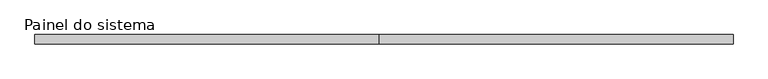
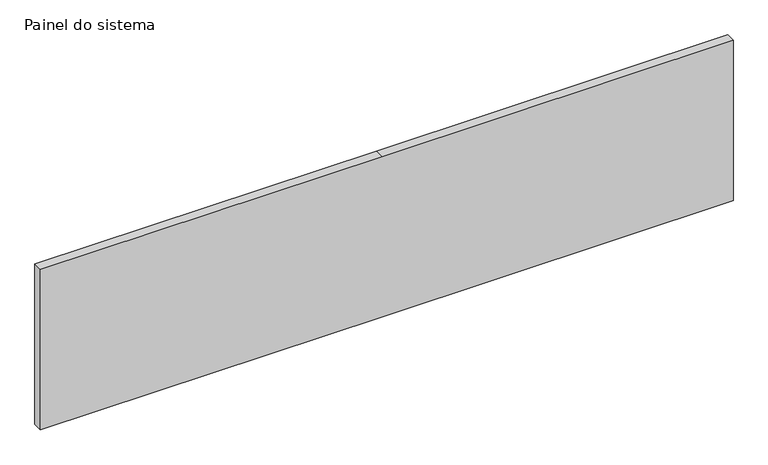
"""IFC4 building model written with IfcOpenShell, lengths in millimetres: plate geometry, Painel do sistema : Envidraçado."""

import ifcopenshell
import ifcopenshell.guid

model = None  # the IFC model being written
_history = None  # IfcOwnerHistory: only IFC2X3 demands one
_inside = {}  # id of a spatial element -> (the spatial element, [elements in it])
_under = {}  # id of a project, library or spatial element -> (it, [spatial elements below it])
_declared = {}  # id of a project -> (the project, [libraries it declares])
_typed = {}  # id of a type object -> (the type object, [elements of that type])
_made_of = {}  # id of a material, layer set ... -> (it, [elements and type objects made of it])


def new_model(schema):
    """Start an empty IFC model of exactly this schema.

    Asked for "IFC4X3", IfcOpenShell would pick the latest addendum, in which some entities
    have other attributes; the version numbers below select the first issue.
    IFC2X3 requires an IfcOwnerHistory on every rooted entity: one is made here for all.
    """
    global model, _history
    if schema == "IFC4X3":
        model = ifcopenshell.file(schema_version=(4, 3, 0, 0))
    else:
        model = ifcopenshell.file(schema=schema)
    _inside.clear()
    _under.clear()
    _declared.clear()
    _typed.clear()
    _made_of.clear()
    _history = None
    if model.schema == "IFC2X3":
        org = make("IfcOrganization", Name="unknown")
        user = make(
            "IfcPersonAndOrganization",
            ThePerson=make("IfcPerson", FamilyName="unknown"),
            TheOrganization=org,
        )
        app = make(
            "IfcApplication",
            ApplicationDeveloper=org,
            Version="unknown",
            ApplicationFullName="unknown",
            ApplicationIdentifier="unknown",
        )
        _history = make(
            "IfcOwnerHistory",
            OwningUser=user,
            OwningApplication=app,
            ChangeAction="ADDED",
            CreationDate=0,
        )
    return model


def make(cls, **values):
    """One entity of the class cls with the attributes given. An attribute that is None is left unset."""
    return model.create_entity(
        cls, **{name: value for name, value in values.items() if value is not None}
    )


def rooted(cls, **values):
    """An entity with a GlobalId (a new one), such as an element, a storey or a relation."""
    return make(cls, GlobalId=ifcopenshell.guid.new(), OwnerHistory=_history, **values)


def si_unit(unit_type, name, prefix=None):
    """IfcSIUnit, for example si_unit("LENGTHUNIT", "METRE", prefix="MILLI")."""
    return make("IfcSIUnit", UnitType=unit_type, Prefix=prefix, Name=name)


def assignment(units):
    """IfcUnitAssignment: the units of a project."""
    return None if units is None else make("IfcUnitAssignment", Units=units)


def point(xyz):
    """IfcCartesianPoint."""
    return None if xyz is None else make("IfcCartesianPoint", Coordinates=xyz)


def direction(xyz):
    """IfcDirection."""
    return None if xyz is None else make("IfcDirection", DirectionRatios=xyz)


def frame(location, z_axis=None, x_axis=None):
    """IfcAxis2Placement3D, a coordinate frame: its origin and axes. An axis left out is left unset."""
    return make(
        "IfcAxis2Placement3D",
        Location=point(location),
        Axis=direction(z_axis),
        RefDirection=direction(x_axis),
    )


def origin():
    """The frame at (0, 0, 0) with its axes left unset."""
    return frame((0.0, 0.0, 0.0))


def place(relative_to, where):
    """IfcLocalPlacement: puts the frame where relative to a parent placement (None: the world)."""
    return make(
        "IfcLocalPlacement", PlacementRelTo=relative_to, RelativePlacement=where
    )


def context(
    kind, dimensions, precision=None, world=None, true_north=None, identifier=None
):
    """IfcGeometricRepresentationContext, for example the 3D "Model" context."""
    return make(
        "IfcGeometricRepresentationContext",
        ContextIdentifier=identifier,
        ContextType=kind,
        CoordinateSpaceDimension=dimensions,
        Precision=precision,
        WorldCoordinateSystem=world,
        TrueNorth=true_north,
    )


def project(units=None, contexts=None):
    """IfcProject with its units and contexts."""
    return rooted(
        "IfcProject",
        Name="project",
        RepresentationContexts=contexts,
        UnitsInContext=assignment(units),
    )


def spatial(cls, under=None, at=None, **own):
    """A site, building, storey or space (cls), placed at a placement, below another one or the project."""
    s = rooted(cls, ObjectPlacement=at, **own)
    if under is not None:
        _under.setdefault(under.id(), (under, []))[1].append(s)
    return s


def polyline(points):
    """IfcPolyline through the points."""
    return make("IfcPolyline", Points=[point(p) for p in points])


def outline(outer, holes=None, kind="AREA"):
    """IfcArbitraryClosedProfileDef: a profile drawn as a closed curve; with holes, ...WithVoids."""
    if holes is None:
        return make("IfcArbitraryClosedProfileDef", ProfileType=kind, OuterCurve=outer)
    return make(
        "IfcArbitraryProfileDefWithVoids",
        ProfileType=kind,
        OuterCurve=outer,
        InnerCurves=holes,
    )


def extrude(swept, where, along, depth):
    """IfcExtrudedAreaSolid: the profile swept, set in the frame where, extruded along a direction by depth."""
    return make(
        "IfcExtrudedAreaSolid",
        SweptArea=swept,
        Position=where,
        ExtrudedDirection=direction(along),
        Depth=depth,
    )


def shape(context_of_items, identifier, shape_type, items):
    """IfcShapeRepresentation: the items that make up one representation, for example the "Body"."""
    return make(
        "IfcShapeRepresentation",
        ContextOfItems=context_of_items,
        RepresentationIdentifier=identifier,
        RepresentationType=shape_type,
        Items=items,
    )


def source(mapping_origin, context_of_items, identifier, shape_type, items):
    """IfcRepresentationMap: a shape defined once, which mapped items show again and again."""
    return make(
        "IfcRepresentationMap",
        MappingOrigin=mapping_origin,
        MappedRepresentation=shape(context_of_items, identifier, shape_type, items),
    )


def transform(
    local_origin,
    x_axis=None,
    y_axis=None,
    z_axis=None,
    scale=None,
    scale2=None,
    scale3=None,
    uniform=True,
):
    """IfcCartesianTransformationOperator3D, or its non-uniform kind. x_axis, y_axis, z_axis: its Axis1, 2, 3."""
    if uniform:
        return make(
            "IfcCartesianTransformationOperator3D",
            Axis1=direction(x_axis),
            Axis2=direction(y_axis),
            LocalOrigin=point(local_origin),
            Scale=scale,
            Axis3=direction(z_axis),
        )
    return make(
        "IfcCartesianTransformationOperator3DnonUniform",
        Axis1=direction(x_axis),
        Axis2=direction(y_axis),
        LocalOrigin=point(local_origin),
        Scale=scale,
        Axis3=direction(z_axis),
        Scale2=scale2,
        Scale3=scale3,
    )


def mapped(mapping_source, mapping_target):
    """IfcMappedItem: shows the shape of a source again, moved by a transform."""
    return make(
        "IfcMappedItem", MappingSource=mapping_source, MappingTarget=mapping_target
    )


def made_of(thing, what):
    """Note that an element or type object is made of a material, layer set ...; save() writes the relation."""
    if what is not None:
        _made_of.setdefault(what.id(), (what, []))[1].append(thing)
    return thing


def element(
    cls,
    number,
    at=None,
    inside=None,
    cuts=None,
    type_object=None,
    material=None,
    context=None,
    identifier="Body",
    shape_type=None,
    held_by="IfcProductDefinitionShape",
    body=None,
    shapes=None,
    **own,
):
    """One element of the class cls, such as IfcWall. Its Tag is "e" and its number.

    at: its placement. inside: the storey or other place that contains it. cuts: it is an
    opening in that element (IfcRelVoidsElement). A single representation is given by context,
    identifier, shape_type and body (its items); several are given by shapes. held_by: the class
    of the entity that holds the representations. save() writes the other relations.
    """
    e = rooted(cls, Tag="e%d" % number, ObjectPlacement=at, **own)
    if body is not None:
        shapes = [shape(context, identifier, shape_type, body)]
    if shapes is not None:
        e.Representation = make(held_by, Representations=shapes)
    if inside is not None:
        _inside.setdefault(inside.id(), (inside, []))[1].append(e)
    if cuts is not None:
        rooted(
            "IfcRelVoidsElement", RelatingBuildingElement=cuts, RelatedOpeningElement=e
        )
    if type_object is not None:
        _typed.setdefault(type_object.id(), (type_object, []))[1].append(e)
    return made_of(e, material)


def aggregate(whole, parts):
    """IfcRelAggregates: a whole, such as a stair, and the parts it consists of."""
    return rooted("IfcRelAggregates", RelatingObject=whole, RelatedObjects=parts)


def save(model, path):
    """Write the relations noted so far, then the file.

    IfcRelAggregates (storeys below a building ...), IfcRelContainedInSpatialStructure (elements
    in a storey), IfcRelDefinesByType, IfcRelAssociatesMaterial and IfcRelDeclares: one each for
    every whole, place, type object, material and project.
    """
    for whole, parts in _under.values():
        aggregate(whole, parts)
    for where, things in _inside.values():
        rooted(
            "IfcRelContainedInSpatialStructure",
            RelatedElements=things,
            RelatingStructure=where,
        )
    for kind, things in _typed.values():
        rooted("IfcRelDefinesByType", RelatedObjects=things, RelatingType=kind)
    for what, things in _made_of.values():
        rooted("IfcRelAssociatesMaterial", RelatedObjects=things, RelatingMaterial=what)
    for by, libraries in _declared.values():
        rooted("IfcRelDeclares", RelatingContext=by, RelatedDefinitions=libraries)
    model.write(path)


def painel_do_sistema_ef095440(model_context):
    return source(origin(), model_context, "Body", "SweptSolid", [
        extrude(outline(polyline([(0.0, -918.5166667), (0.0, -12.4999998), (0.0, 918.5166667), (450.0, 918.5166667), (450.0, -12.4999998), (450.0, -918.5166667), (0.0, -918.5166667)])), frame((0.0, 24.5, 0.0), z_axis=(0.0, 1.0, 0.0), x_axis=(0.0, 0.0, 1.0)), (0.0, 0.0, 1.0), 25.0),
    ])


if __name__ == "__main__":
    model = new_model("IFC4")
    model_context = context("Model", 3, world=origin())
    ifc_project = project(units=[si_unit("LENGTHUNIT", "METRE", prefix="MILLI")], contexts=[model_context])
    site = spatial("IfcSite", under=ifc_project)
    building = spatial("IfcBuilding", under=site)
    placement = place(None, origin())
    painel_do_sistema_shape = painel_do_sistema_ef095440(model_context)
    element("IfcPlate", 1, ObjectType="Painel do sistema : Envidraçado", at=placement, inside=building, context=model_context, shape_type="MappedRepresentation", body=[
        mapped(painel_do_sistema_shape, transform((0.0, 0.0, 0.0), x_axis=(1.0, 0.0, 0.0), y_axis=(0.0, 1.0, 0.0), z_axis=(0.0, 0.0, 1.0))),
    ])
    save(model, "model.ifc")

# Revit data of these elements
# Type "Painel do sistema : Envidraçado"
#   Construction Type Id = "GSP4R"
#   Analytic Construction = "Vidraça única Pilkington 1/8 pol"
#   Visual Light Transmittance = 0.9
#   Solar Heat Gain Coefficient = 0.86
#   Heat Transfer Coefficient (U) = 6.7069 W/(m²·K)
# Element 1 (IfcPlate, "Painel do sistema : Envidraçado")
#   Materials on its faces: ".VIDRO GENÉRICO"
# Materials
#   ".VIDRO GENÉRICO": class ".CC_VIDRO", colour RGB 0 128 192, transparency 0.9, Description = "Vidro comum", Cost = 0
